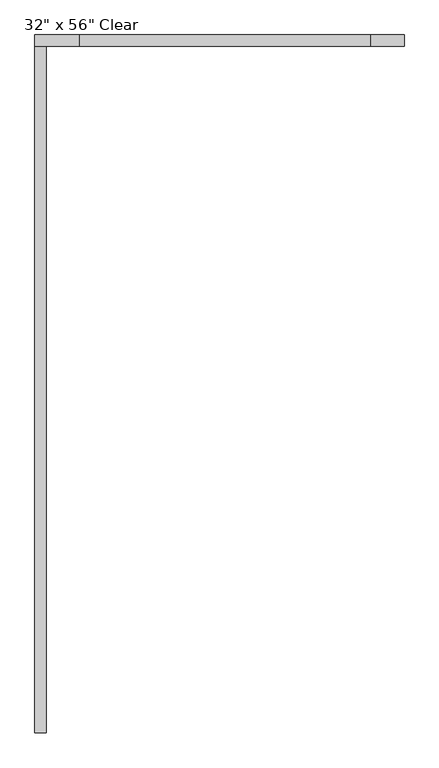
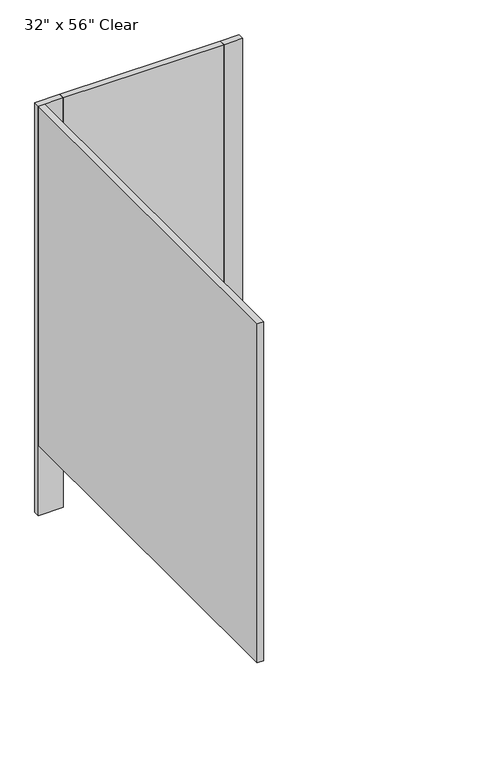
"""IFC4 building model written with IfcOpenShell, lengths in millimetres: proxy geometry."""

import ifcopenshell
import ifcopenshell.guid

model = None  # the IFC model being written
_history = None  # IfcOwnerHistory: only IFC2X3 demands one
_inside = {}  # id of a spatial element -> (the spatial element, [elements in it])
_under = {}  # id of a project, library or spatial element -> (it, [spatial elements below it])
_declared = {}  # id of a project -> (the project, [libraries it declares])
_typed = {}  # id of a type object -> (the type object, [elements of that type])
_made_of = {}  # id of a material, layer set ... -> (it, [elements and type objects made of it])


def new_model(schema):
    """Start an empty IFC model of exactly this schema.

    Asked for "IFC4X3", IfcOpenShell would pick the latest addendum, in which some entities
    have other attributes; the version numbers below select the first issue.
    IFC2X3 requires an IfcOwnerHistory on every rooted entity: one is made here for all.
    """
    global model, _history
    if schema == "IFC4X3":
        model = ifcopenshell.file(schema_version=(4, 3, 0, 0))
    else:
        model = ifcopenshell.file(schema=schema)
    _inside.clear()
    _under.clear()
    _declared.clear()
    _typed.clear()
    _made_of.clear()
    _history = None
    if model.schema == "IFC2X3":
        org = make("IfcOrganization", Name="unknown")
        user = make(
            "IfcPersonAndOrganization",
            ThePerson=make("IfcPerson", FamilyName="unknown"),
            TheOrganization=org,
        )
        app = make(
            "IfcApplication",
            ApplicationDeveloper=org,
            Version="unknown",
            ApplicationFullName="unknown",
            ApplicationIdentifier="unknown",
        )
        _history = make(
            "IfcOwnerHistory",
            OwningUser=user,
            OwningApplication=app,
            ChangeAction="ADDED",
            CreationDate=0,
        )
    return model


def make(cls, **values):
    """One entity of the class cls with the attributes given. An attribute that is None is left unset."""
    return model.create_entity(
        cls, **{name: value for name, value in values.items() if value is not None}
    )


def rooted(cls, **values):
    """An entity with a GlobalId (a new one), such as an element, a storey or a relation."""
    return make(cls, GlobalId=ifcopenshell.guid.new(), OwnerHistory=_history, **values)


def si_unit(unit_type, name, prefix=None):
    """IfcSIUnit, for example si_unit("LENGTHUNIT", "METRE", prefix="MILLI")."""
    return make("IfcSIUnit", UnitType=unit_type, Prefix=prefix, Name=name)


def assignment(units):
    """IfcUnitAssignment: the units of a project."""
    return None if units is None else make("IfcUnitAssignment", Units=units)


def point(xyz):
    """IfcCartesianPoint."""
    return None if xyz is None else make("IfcCartesianPoint", Coordinates=xyz)


def direction(xyz):
    """IfcDirection."""
    return None if xyz is None else make("IfcDirection", DirectionRatios=xyz)


def frame(location, z_axis=None, x_axis=None):
    """IfcAxis2Placement3D, a coordinate frame: its origin and axes. An axis left out is left unset."""
    return make(
        "IfcAxis2Placement3D",
        Location=point(location),
        Axis=direction(z_axis),
        RefDirection=direction(x_axis),
    )


def origin():
    """The frame at (0, 0, 0) with its axes left unset."""
    return frame((0.0, 0.0, 0.0))


def origin_with_axes():
    """The frame at (0, 0, 0) with the z axis (0, 0, 1) and the x axis (1, 0, 0) written out."""
    return frame((0.0, 0.0, 0.0), z_axis=(0.0, 0.0, 1.0), x_axis=(1.0, 0.0, 0.0))


def place(relative_to, where):
    """IfcLocalPlacement: puts the frame where relative to a parent placement (None: the world)."""
    return make(
        "IfcLocalPlacement", PlacementRelTo=relative_to, RelativePlacement=where
    )


def context(
    kind, dimensions, precision=None, world=None, true_north=None, identifier=None
):
    """IfcGeometricRepresentationContext, for example the 3D "Model" context."""
    return make(
        "IfcGeometricRepresentationContext",
        ContextIdentifier=identifier,
        ContextType=kind,
        CoordinateSpaceDimension=dimensions,
        Precision=precision,
        WorldCoordinateSystem=world,
        TrueNorth=true_north,
    )


def project(units=None, contexts=None):
    """IfcProject with its units and contexts."""
    return rooted(
        "IfcProject",
        Name="project",
        RepresentationContexts=contexts,
        UnitsInContext=assignment(units),
    )


def spatial(cls, under=None, at=None, **own):
    """A site, building, storey or space (cls), placed at a placement, below another one or the project."""
    s = rooted(cls, ObjectPlacement=at, **own)
    if under is not None:
        _under.setdefault(under.id(), (under, []))[1].append(s)
    return s


def polyline(points):
    """IfcPolyline through the points."""
    return make("IfcPolyline", Points=[point(p) for p in points])


def outline(outer, holes=None, kind="AREA"):
    """IfcArbitraryClosedProfileDef: a profile drawn as a closed curve; with holes, ...WithVoids."""
    if holes is None:
        return make("IfcArbitraryClosedProfileDef", ProfileType=kind, OuterCurve=outer)
    return make(
        "IfcArbitraryProfileDefWithVoids",
        ProfileType=kind,
        OuterCurve=outer,
        InnerCurves=holes,
    )


def extrude(swept, where, along, depth):
    """IfcExtrudedAreaSolid: the profile swept, set in the frame where, extruded along a direction by depth."""
    return make(
        "IfcExtrudedAreaSolid",
        SweptArea=swept,
        Position=where,
        ExtrudedDirection=direction(along),
        Depth=depth,
    )


def shape(context_of_items, identifier, shape_type, items):
    """IfcShapeRepresentation: the items that make up one representation, for example the "Body"."""
    return make(
        "IfcShapeRepresentation",
        ContextOfItems=context_of_items,
        RepresentationIdentifier=identifier,
        RepresentationType=shape_type,
        Items=items,
    )


def source(mapping_origin, context_of_items, identifier, shape_type, items):
    """IfcRepresentationMap: a shape defined once, which mapped items show again and again."""
    return make(
        "IfcRepresentationMap",
        MappingOrigin=mapping_origin,
        MappedRepresentation=shape(context_of_items, identifier, shape_type, items),
    )


def transform(
    local_origin,
    x_axis=None,
    y_axis=None,
    z_axis=None,
    scale=None,
    scale2=None,
    scale3=None,
    uniform=True,
):
    """IfcCartesianTransformationOperator3D, or its non-uniform kind. x_axis, y_axis, z_axis: its Axis1, 2, 3."""
    if uniform:
        return make(
            "IfcCartesianTransformationOperator3D",
            Axis1=direction(x_axis),
            Axis2=direction(y_axis),
            LocalOrigin=point(local_origin),
            Scale=scale,
            Axis3=direction(z_axis),
        )
    return make(
        "IfcCartesianTransformationOperator3DnonUniform",
        Axis1=direction(x_axis),
        Axis2=direction(y_axis),
        LocalOrigin=point(local_origin),
        Scale=scale,
        Axis3=direction(z_axis),
        Scale2=scale2,
        Scale3=scale3,
    )


def mapped(mapping_source, mapping_target):
    """IfcMappedItem: shows the shape of a source again, moved by a transform."""
    return make(
        "IfcMappedItem", MappingSource=mapping_source, MappingTarget=mapping_target
    )


def made_of(thing, what):
    """Note that an element or type object is made of a material, layer set ...; save() writes the relation."""
    if what is not None:
        _made_of.setdefault(what.id(), (what, []))[1].append(thing)
    return thing


def element(
    cls,
    number,
    at=None,
    inside=None,
    cuts=None,
    type_object=None,
    material=None,
    context=None,
    identifier="Body",
    shape_type=None,
    held_by="IfcProductDefinitionShape",
    body=None,
    shapes=None,
    **own,
):
    """One element of the class cls, such as IfcWall. Its Tag is "e" and its number.

    at: its placement. inside: the storey or other place that contains it. cuts: it is an
    opening in that element (IfcRelVoidsElement). A single representation is given by context,
    identifier, shape_type and body (its items); several are given by shapes. held_by: the class
    of the entity that holds the representations. save() writes the other relations.
    """
    e = rooted(cls, Tag="e%d" % number, ObjectPlacement=at, **own)
    if body is not None:
        shapes = [shape(context, identifier, shape_type, body)]
    if shapes is not None:
        e.Representation = make(held_by, Representations=shapes)
    if inside is not None:
        _inside.setdefault(inside.id(), (inside, []))[1].append(e)
    if cuts is not None:
        rooted(
            "IfcRelVoidsElement", RelatingBuildingElement=cuts, RelatedOpeningElement=e
        )
    if type_object is not None:
        _typed.setdefault(type_object.id(), (type_object, []))[1].append(e)
    return made_of(e, material)


def aggregate(whole, parts):
    """IfcRelAggregates: a whole, such as a stair, and the parts it consists of."""
    return rooted("IfcRelAggregates", RelatingObject=whole, RelatedObjects=parts)


def save(model, path):
    """Write the relations noted so far, then the file.

    IfcRelAggregates (storeys below a building ...), IfcRelContainedInSpatialStructure (elements
    in a storey), IfcRelDefinesByType, IfcRelAssociatesMaterial and IfcRelDeclares: one each for
    every whole, place, type object, material and project.
    """
    for whole, parts in _under.values():
        aggregate(whole, parts)
    for where, things in _inside.values():
        rooted(
            "IfcRelContainedInSpatialStructure",
            RelatedElements=things,
            RelatingStructure=where,
        )
    for kind, things in _typed.values():
        rooted("IfcRelDefinesByType", RelatedObjects=things, RelatingType=kind)
    for what, things in _made_of.values():
        rooted("IfcRelAssociatesMaterial", RelatedObjects=things, RelatingMaterial=what)
    for by, libraries in _declared.values():
        rooted("IfcRelDeclares", RelatingContext=by, RelatedDefinitions=libraries)
    model.write(path)


def proxy_86d28e76(model_context):
    return source(origin(), model_context, "Body", "SweptSolid", [
        extrude(outline(polyline([(735.1031538, 1646.2375), (735.1031538, 1620.8375), (74.7031538, 1620.8375), (74.7031538, 1646.2375), (735.1031538, 1646.2375)])), frame((0.0, 0.0, 304.8), z_axis=(0.0, 0.0, 1.0), x_axis=(1.0, 0.0, 0.0)), (0.0, 0.0, 1.0), 1473.2),
        extrude(outline(polyline([(74.7031538, 1646.2375), (74.7031538, 1620.8375), (-26.8968462, 1620.8375), (-26.8968462, 1646.2375), (74.7031538, 1646.2375)])), origin_with_axes(), (0.0, 0.0, 1.0), 1778.0),
        extrude(outline(polyline([(811.3031538, 1646.2375), (811.3031538, 1620.8375), (735.1031538, 1620.8375), (735.1031538, 1646.2375), (811.3031538, 1646.2375)])), origin_with_axes(), (0.0, 0.0, 1.0), 1778.0),
        extrude(outline(polyline([(-26.8968462, 1620.8375), (-1.4968462, 1620.8375), (-1.4968462, 63.5), (-26.8968462, 63.5), (-26.8968462, 1620.8375)])), frame((0.0, 0.0, 304.8), z_axis=(0.0, 0.0, 1.0), x_axis=(1.0, 0.0, 0.0)), (0.0, 0.0, 1.0), 1473.2),
    ])


if __name__ == "__main__":
    model = new_model("IFC4")
    model_context = context("Model", 3, world=origin())
    ifc_project = project(units=[si_unit("LENGTHUNIT", "METRE", prefix="MILLI")], contexts=[model_context])
    site = spatial("IfcSite", under=ifc_project)
    building = spatial("IfcBuilding", under=site)
    placement = place(None, origin())
    proxy_shape = proxy_86d28e76(model_context)
    element("IfcBuildingElementProxy", 1, Name="Toilet Stall-3D w Toilet : 32\" x 56\" Clear", ObjectType="Toilet Stall-3D w Toilet : 32\" x 56\" Clear", at=placement, inside=building, context=model_context, shape_type="MappedRepresentation", body=[
        mapped(proxy_shape, transform((0.0, 0.0, 0.0), x_axis=(1.0, 0.0, 0.0), y_axis=(0.0, 1.0, 0.0), z_axis=(0.0, 0.0, 1.0))),
    ])
    save(model, "model.ifc")

# Revit data of these elements
# Type "Toilet Stall-3D w Toilet : 32\" x 56\" Clear"
#   Assembly Code = "C1030100"
#   Door Width = 2' - 2"
#   Length = 4' - 8"
#   Width = 2' - 8"
#   Toilet Partition Material = Toilet Partition
#   Default Elevation = 0
# Element 1 (IfcBuildingElementProxy, "Toilet Stall-3D w Toilet : 32\" x 56\" Clear")
#   Materials on its faces: "Toilet Partition"
# Materials
#   "Toilet Partition": class "Unassigned", colour RGB 0 181 188, transparency 0
